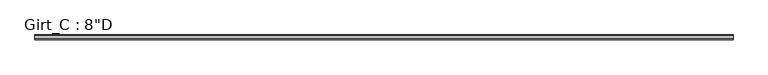
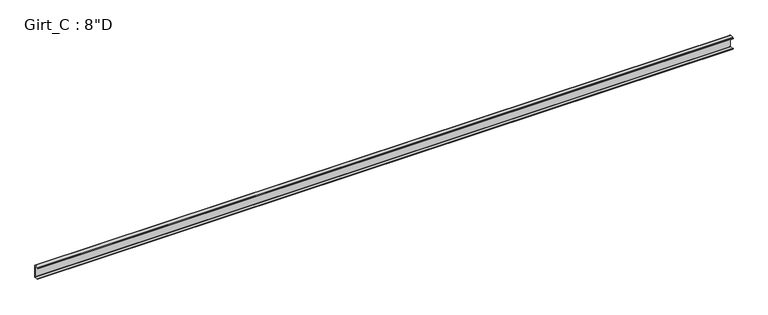
"""IFC4 building model written with IfcOpenShell, lengths in millimetres: beam geometry."""

from ifc_helpers import new_model, si_unit, point, frame, frame_2d, origin, place, context, project, spatial, polyline, circle_curve, trimmed, segment, composite_curve, outline, extrude, source, transform, mapped, element, save


def beam_1a248c92(model_context):
    return source(origin(), model_context, "Body", "SweptSolid", [
        extrude(outline(composite_curve([segment(polyline([(-63.5, 101.6), (-3.3734375, 101.6)]), True, "CONTINUOUS"), segment(trimmed(circle_curve(frame_2d((-3.3734375, 96.8375)), 4.7625), [point((-3.3734375, 101.6))], [point((1.3890625, 96.8375))], False, "CARTESIAN"), True, "CONTINUOUS"), segment(polyline([(1.3890625, 96.8375), (1.3890625, -96.8375)]), True, "CONTINUOUS"), segment(trimmed(circle_curve(frame_2d((-3.3734375, -96.8375)), 4.7625), [point((1.3890625, -96.8375))], [point((-3.3734375, -101.6))], False, "CARTESIAN"), True, "CONTINUOUS"), segment(polyline([(-3.3734375, -101.6), (-63.5, -101.6), (-75.745104, -87.0068534), (-73.6169367, -85.221109), (-62.204539, -98.821875), (-3.2694106, -98.821875)]), True, "CONTINUOUS"), segment(trimmed(circle_curve(frame_2d((-3.3748024, -96.8389339)), 1.9857399), [point((-3.2694106, -98.821875))], [point((-1.3890625, -96.8389339))], True, "CARTESIAN"), True, "CONTINUOUS"), segment(polyline([(-1.3890625, -96.8389339), (-1.3890625, 96.8381931)]), True, "CONTINUOUS"), segment(trimmed(circle_curve(frame_2d((-3.3741066, 96.8381931)), 1.9850441), [point((-1.3890625, 96.8381931))], [point((-3.3005807, 98.821875))], True, "CARTESIAN"), True, "CONTINUOUS"), segment(polyline([(-3.3005807, 98.821875), (-62.204539, 98.821875), (-73.6169367, 85.221109), (-75.745104, 87.0068534), (-63.5, 101.6)]), True, "CONTINUOUS")], self_intersect=False)), frame((-5562.6, 0.0, 0.0), z_axis=(1.0, 0.0, 0.0), x_axis=(0.0, 1.0, 0.0)), (0.0, 0.0, 1.0), 11280.775),
    ])


if __name__ == "__main__":
    model = new_model("IFC4")
    model_context = context("Model", 3, world=origin())
    ifc_project = project(units=[si_unit("LENGTHUNIT", "METRE", prefix="MILLI")], contexts=[model_context])
    site = spatial("IfcSite", under=ifc_project)
    building = spatial("IfcBuilding", under=site)
    placement = place(None, origin())
    beam_shape = beam_1a248c92(model_context)
    element("IfcBeam", 1, ObjectType="Girt_C : 8\"D", at=placement, inside=building, context=model_context, shape_type="MappedRepresentation", body=[
        mapped(beam_shape, transform((0.0, 0.0, 0.0), x_axis=(1.0, 0.0, 0.0), y_axis=(0.0, 1.0, 0.0), z_axis=(0.0, 0.0, 1.0))),
    ])
    save(model, "model.ifc")

# Revit data of these elements
# Type "Girt_C : 8\"D"
#   Web_Thickness = 0' - 0 7/64"
#   Length [instance default] = 10' - 0"
#   Leg_1 = 0' - 2 1/2"
#   Height = 0' - 8"
#   Structural Material [instance default] = none
# Element 1 (IfcBeam, "Girt_C : 8\"D")
#   Structural Material = Steel
#   Materials on its faces: "Steel"
# Materials
#   "Steel": class "Metal", colour RGB 118 118 114, transparency 0, Description = "Steel, mill finish", Cost = 0
